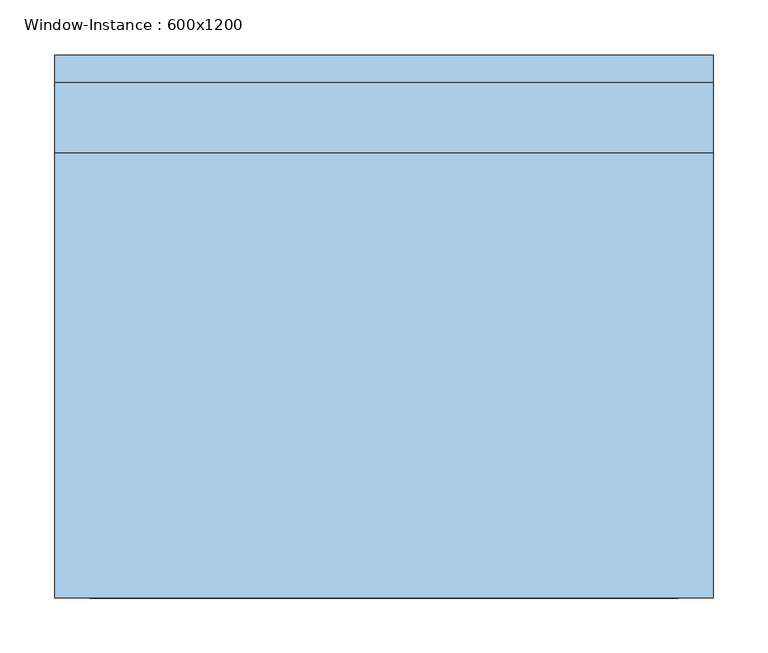
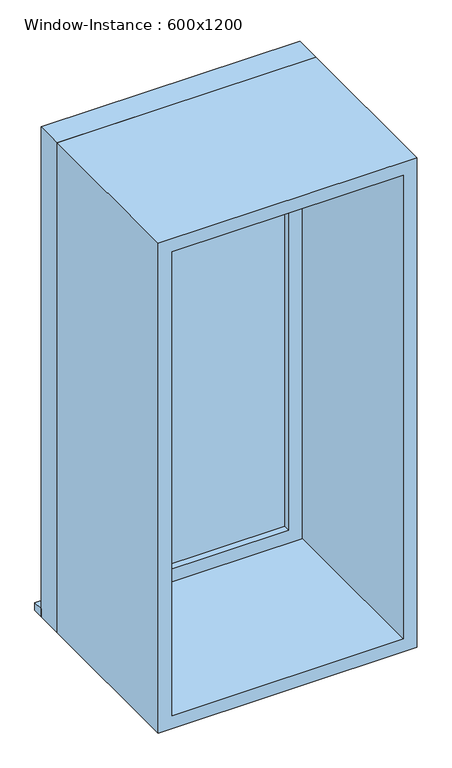
"""IFC4 building model written with IfcOpenShell, lengths in millimetres: window geometry, Window-Instance : 600x1200."""

from ifc_helpers import new_model, si_unit, frame, origin, place, context, project, spatial, polyline, outline, extrude, source, transform, mapped, element, save


def window_instance_600x1200_e1fbdb17(model_context):
    return source(origin(), model_context, "Body", "SweptSolid", [
        extrude(outline(polyline([(-338.1, 260.4), (261.9, 260.4), (261.9, 235.0), (-338.1, 235.0), (-338.1, 260.4)])), frame((0.0, 0.0, 900.0), z_axis=(0.0, 0.0, 1.0), x_axis=(1.0, 0.0, 0.0)), (0.0, 0.0, 1.0), 19.05),
        extrude(outline(polyline([(198.4, 186.425), (-274.6, 186.425), (-274.6, 199.125), (198.4, 199.125), (198.4, 186.425)])), frame((0.0, 0.0, 963.5), z_axis=(0.0, 0.0, 1.0), x_axis=(1.0, 0.0, 0.0)), (0.0, 0.0, 1.0), 1073.0),
        extrude(outline(polyline([(2080.95, -319.05), (919.05, -319.05), (919.05, 242.85), (2080.95, 242.85), (2080.95, -319.05)]), holes=[polyline([(2036.5, -274.6), (2036.5, 198.4), (963.5, 198.4), (963.5, -274.6), (2036.5, -274.6)])]), frame((0.0, 170.55, 0.0), z_axis=(0.0, 1.0, 0.0), x_axis=(0.0, 0.0, 1.0)), (0.0, 0.0, 1.0), 44.45),
        extrude(outline(polyline([(2100.0, -338.1), (900.0, -338.1), (900.0, 261.9), (2100.0, 261.9), (2100.0, -338.1)]), holes=[polyline([(2068.25, -306.35), (2068.25, 230.15), (931.75, 230.15), (931.75, -306.35), (2068.25, -306.35)])]), frame((0.0, -235.0, 0.0), z_axis=(0.0, 1.0, 0.0), x_axis=(0.0, 0.0, 1.0)), (0.0, 0.0, 1.0), 405.55),
        extrude(outline(polyline([(2100.0, 261.9), (2100.0, -338.1), (900.0, -338.1), (900.0, 261.9), (2100.0, 261.9)]), holes=[polyline([(2080.95, 242.85), (919.05, 242.85), (919.05, -319.05), (2080.95, -319.05), (2080.95, 242.85)])]), frame((0.0, 170.55, 0.0), z_axis=(0.0, 1.0, 0.0), x_axis=(0.0, 0.0, 1.0)), (0.0, 0.0, 1.0), 64.45),
    ])


if __name__ == "__main__":
    model = new_model("IFC4")
    model_context = context("Model", 3, world=origin())
    ifc_project = project(units=[si_unit("LENGTHUNIT", "METRE", prefix="MILLI")], contexts=[model_context])
    site = spatial("IfcSite", under=ifc_project)
    building = spatial("IfcBuilding", under=site)
    placement = place(None, origin())
    window_instance_600x1200_shape = window_instance_600x1200_e1fbdb17(model_context)
    element("IfcWindow", 1, ObjectType="Window-Instance : 600x1200", at=placement, inside=building, context=model_context, shape_type="MappedRepresentation", body=[
        mapped(window_instance_600x1200_shape, transform((0.0, 0.0, 0.0), x_axis=(1.0, 0.0, 0.0), y_axis=(0.0, 1.0, 0.0), z_axis=(0.0, 0.0, 1.0))),
    ])
    save(model, "model.ifc")

# Revit data of these elements
# Type "Window-Instance : 600x1200"
#   Type Mark = "7"
#   Construction Type Id = "GSP4R"
#   Assembly Code = "B2020100"
#   Analytic Construction = "1/8 in Pilkington single glazing"
#   Visual Light Transmittance = 0.9
#   Thermal Resistance (R) = 0.149095 (m²·K)/W
#   Solar Heat Gain Coefficient = 0.86
#   Heat Transfer Coefficient (U) = 6.70716 W/(m²·K)
#   Height [instance default] = 1200 mm
#   Default Sill Height = 900 mm
#   Width [instance default] = 600 mm
#   Window Inset = 20 mm
#   Glass Pane Material = WW-EC-GL-Storefront
#   Sash Material = WW-EC-RGB-White
#   Wall Closure = (empty or 0)
# Element 1 (IfcWindow, "Window-Instance : 600x1200")
#   Materials on its faces: "WW-EC-RGB-White", "WW-EC-GL-Storefront"
# Materials
#   "WW-EC-GL-Storefront": class "Glass", colour RGB 236 240 239, transparency 0.85, Description = "Storefront Glass", Cost = 0
#   "WW-EC-RGB-White": class "Generic", colour RGB 255 255 255, transparency 0, Comments = "If region requests off-white, swith asset color to RGB 231-228-220", Description = "Generic Color", Cost = 0
